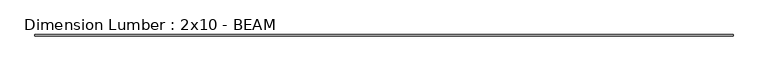
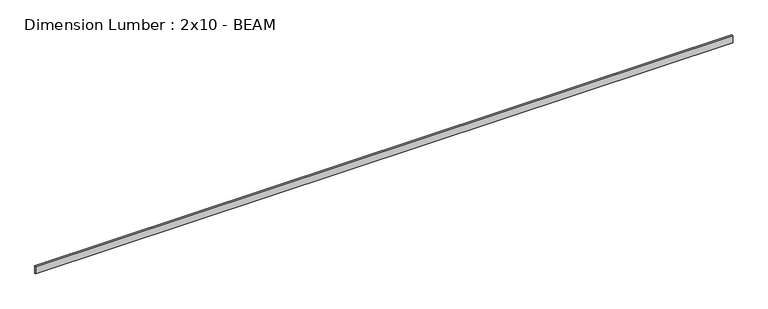
"""IFC4 building model written with IfcOpenShell, lengths in millimetres: beam geometry, Dimension Lumber : 2x10 - BEAM."""

from ifc_helpers import new_model, si_unit, frame, origin, place, context, project, spatial, polyline, outline, extrude, source, transform, mapped, element, save


def dimension_lumber_2x10_beam_967a23c9(model_context):
    return source(origin(), model_context, "Body", "SweptSolid", [
        extrude(outline(polyline([(10614.0994135, 19.05), (10614.0994135, -19.05), (-10776.0244141, -19.05), (-10776.0244141, 19.05), (10614.0994135, 19.05)])), frame((0.0, 0.0, -117.475), z_axis=(0.0, 0.0, 1.0), x_axis=(1.0, 0.0, 0.0)), (0.0, 0.0, 1.0), 234.95),
    ])


if __name__ == "__main__":
    model = new_model("IFC4")
    model_context = context("Model", 3, world=origin())
    ifc_project = project(units=[si_unit("LENGTHUNIT", "METRE", prefix="MILLI")], contexts=[model_context])
    site = spatial("IfcSite", under=ifc_project)
    building = spatial("IfcBuilding", under=site)
    placement = place(None, origin())
    dimension_lumber_2x10_beam_shape = dimension_lumber_2x10_beam_967a23c9(model_context)
    element("IfcBeam", 1, ObjectType="Dimension Lumber : 2x10 - BEAM", at=placement, inside=building, context=model_context, shape_type="MappedRepresentation", body=[
        mapped(dimension_lumber_2x10_beam_shape, transform((0.0, 0.0, 0.0), x_axis=(1.0, 0.0, 0.0), y_axis=(0.0, 1.0, 0.0), z_axis=(0.0, 0.0, 1.0))),
    ])
    save(model, "model.ifc")

# Revit data of these elements
# Type "Dimension Lumber : 2x10 - BEAM"
#   Assembly Code = "B10"
#   A = 0.0755556 SF
#   Length [instance default] = 5' - 0"
#   b = 0' - 1 1/2"
#   d = 0' - 9 1/4"
#   Structural Material = (3) SISTERED 2X10s AT BEAM
# Element 1 (IfcBeam, "Dimension Lumber : 2x10 - BEAM")
#   Materials on its faces: "(3) SISTERED 2X10s AT BEAM"
# Materials
#   "(3) SISTERED 2X10s AT BEAM": class "Wood", colour RGB 234 198 147, transparency 0, Description = "Pinus Echinata", Cost = 0
